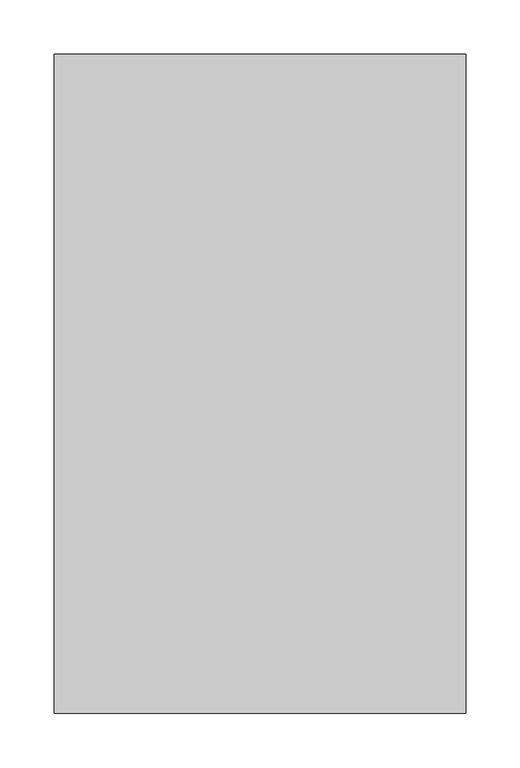
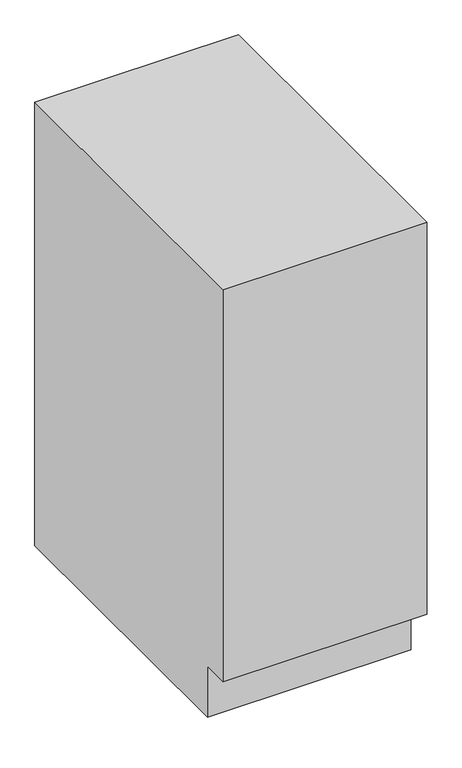
"""IFC4 building model written with IfcOpenShell, lengths in millimetres: furniture geometry, Cabinet, Base Integrated Trash Single-NON-COLLECTUS : -."""

import ifcopenshell
import ifcopenshell.guid

model = None  # the IFC model being written
_history = None  # IfcOwnerHistory: only IFC2X3 demands one
_inside = {}  # id of a spatial element -> (the spatial element, [elements in it])
_under = {}  # id of a project, library or spatial element -> (it, [spatial elements below it])
_declared = {}  # id of a project -> (the project, [libraries it declares])
_typed = {}  # id of a type object -> (the type object, [elements of that type])
_made_of = {}  # id of a material, layer set ... -> (it, [elements and type objects made of it])


def new_model(schema):
    """Start an empty IFC model of exactly this schema.

    Asked for "IFC4X3", IfcOpenShell would pick the latest addendum, in which some entities
    have other attributes; the version numbers below select the first issue.
    IFC2X3 requires an IfcOwnerHistory on every rooted entity: one is made here for all.
    """
    global model, _history
    if schema == "IFC4X3":
        model = ifcopenshell.file(schema_version=(4, 3, 0, 0))
    else:
        model = ifcopenshell.file(schema=schema)
    _inside.clear()
    _under.clear()
    _declared.clear()
    _typed.clear()
    _made_of.clear()
    _history = None
    if model.schema == "IFC2X3":
        org = make("IfcOrganization", Name="unknown")
        user = make(
            "IfcPersonAndOrganization",
            ThePerson=make("IfcPerson", FamilyName="unknown"),
            TheOrganization=org,
        )
        app = make(
            "IfcApplication",
            ApplicationDeveloper=org,
            Version="unknown",
            ApplicationFullName="unknown",
            ApplicationIdentifier="unknown",
        )
        _history = make(
            "IfcOwnerHistory",
            OwningUser=user,
            OwningApplication=app,
            ChangeAction="ADDED",
            CreationDate=0,
        )
    return model


def make(cls, **values):
    """One entity of the class cls with the attributes given. An attribute that is None is left unset."""
    return model.create_entity(
        cls, **{name: value for name, value in values.items() if value is not None}
    )


def rooted(cls, **values):
    """An entity with a GlobalId (a new one), such as an element, a storey or a relation."""
    return make(cls, GlobalId=ifcopenshell.guid.new(), OwnerHistory=_history, **values)


def si_unit(unit_type, name, prefix=None):
    """IfcSIUnit, for example si_unit("LENGTHUNIT", "METRE", prefix="MILLI")."""
    return make("IfcSIUnit", UnitType=unit_type, Prefix=prefix, Name=name)


def assignment(units):
    """IfcUnitAssignment: the units of a project."""
    return None if units is None else make("IfcUnitAssignment", Units=units)


def point(xyz):
    """IfcCartesianPoint."""
    return None if xyz is None else make("IfcCartesianPoint", Coordinates=xyz)


def direction(xyz):
    """IfcDirection."""
    return None if xyz is None else make("IfcDirection", DirectionRatios=xyz)


def frame(location, z_axis=None, x_axis=None):
    """IfcAxis2Placement3D, a coordinate frame: its origin and axes. An axis left out is left unset."""
    return make(
        "IfcAxis2Placement3D",
        Location=point(location),
        Axis=direction(z_axis),
        RefDirection=direction(x_axis),
    )


def origin():
    """The frame at (0, 0, 0) with its axes left unset."""
    return frame((0.0, 0.0, 0.0))


def place(relative_to, where):
    """IfcLocalPlacement: puts the frame where relative to a parent placement (None: the world)."""
    return make(
        "IfcLocalPlacement", PlacementRelTo=relative_to, RelativePlacement=where
    )


def context(
    kind, dimensions, precision=None, world=None, true_north=None, identifier=None
):
    """IfcGeometricRepresentationContext, for example the 3D "Model" context."""
    return make(
        "IfcGeometricRepresentationContext",
        ContextIdentifier=identifier,
        ContextType=kind,
        CoordinateSpaceDimension=dimensions,
        Precision=precision,
        WorldCoordinateSystem=world,
        TrueNorth=true_north,
    )


def project(units=None, contexts=None):
    """IfcProject with its units and contexts."""
    return rooted(
        "IfcProject",
        Name="project",
        RepresentationContexts=contexts,
        UnitsInContext=assignment(units),
    )


def spatial(cls, under=None, at=None, **own):
    """A site, building, storey or space (cls), placed at a placement, below another one or the project."""
    s = rooted(cls, ObjectPlacement=at, **own)
    if under is not None:
        _under.setdefault(under.id(), (under, []))[1].append(s)
    return s


def polyline(points):
    """IfcPolyline through the points."""
    return make("IfcPolyline", Points=[point(p) for p in points])


def outline(outer, holes=None, kind="AREA"):
    """IfcArbitraryClosedProfileDef: a profile drawn as a closed curve; with holes, ...WithVoids."""
    if holes is None:
        return make("IfcArbitraryClosedProfileDef", ProfileType=kind, OuterCurve=outer)
    return make(
        "IfcArbitraryProfileDefWithVoids",
        ProfileType=kind,
        OuterCurve=outer,
        InnerCurves=holes,
    )


def extrude(swept, where, along, depth):
    """IfcExtrudedAreaSolid: the profile swept, set in the frame where, extruded along a direction by depth."""
    return make(
        "IfcExtrudedAreaSolid",
        SweptArea=swept,
        Position=where,
        ExtrudedDirection=direction(along),
        Depth=depth,
    )


def shape(context_of_items, identifier, shape_type, items):
    """IfcShapeRepresentation: the items that make up one representation, for example the "Body"."""
    return make(
        "IfcShapeRepresentation",
        ContextOfItems=context_of_items,
        RepresentationIdentifier=identifier,
        RepresentationType=shape_type,
        Items=items,
    )


def source(mapping_origin, context_of_items, identifier, shape_type, items):
    """IfcRepresentationMap: a shape defined once, which mapped items show again and again."""
    return make(
        "IfcRepresentationMap",
        MappingOrigin=mapping_origin,
        MappedRepresentation=shape(context_of_items, identifier, shape_type, items),
    )


def transform(
    local_origin,
    x_axis=None,
    y_axis=None,
    z_axis=None,
    scale=None,
    scale2=None,
    scale3=None,
    uniform=True,
):
    """IfcCartesianTransformationOperator3D, or its non-uniform kind. x_axis, y_axis, z_axis: its Axis1, 2, 3."""
    if uniform:
        return make(
            "IfcCartesianTransformationOperator3D",
            Axis1=direction(x_axis),
            Axis2=direction(y_axis),
            LocalOrigin=point(local_origin),
            Scale=scale,
            Axis3=direction(z_axis),
        )
    return make(
        "IfcCartesianTransformationOperator3DnonUniform",
        Axis1=direction(x_axis),
        Axis2=direction(y_axis),
        LocalOrigin=point(local_origin),
        Scale=scale,
        Axis3=direction(z_axis),
        Scale2=scale2,
        Scale3=scale3,
    )


def mapped(mapping_source, mapping_target):
    """IfcMappedItem: shows the shape of a source again, moved by a transform."""
    return make(
        "IfcMappedItem", MappingSource=mapping_source, MappingTarget=mapping_target
    )


def made_of(thing, what):
    """Note that an element or type object is made of a material, layer set ...; save() writes the relation."""
    if what is not None:
        _made_of.setdefault(what.id(), (what, []))[1].append(thing)
    return thing


def element(
    cls,
    number,
    at=None,
    inside=None,
    cuts=None,
    type_object=None,
    material=None,
    context=None,
    identifier="Body",
    shape_type=None,
    held_by="IfcProductDefinitionShape",
    body=None,
    shapes=None,
    **own,
):
    """One element of the class cls, such as IfcWall. Its Tag is "e" and its number.

    at: its placement. inside: the storey or other place that contains it. cuts: it is an
    opening in that element (IfcRelVoidsElement). A single representation is given by context,
    identifier, shape_type and body (its items); several are given by shapes. held_by: the class
    of the entity that holds the representations. save() writes the other relations.
    """
    e = rooted(cls, Tag="e%d" % number, ObjectPlacement=at, **own)
    if body is not None:
        shapes = [shape(context, identifier, shape_type, body)]
    if shapes is not None:
        e.Representation = make(held_by, Representations=shapes)
    if inside is not None:
        _inside.setdefault(inside.id(), (inside, []))[1].append(e)
    if cuts is not None:
        rooted(
            "IfcRelVoidsElement", RelatingBuildingElement=cuts, RelatedOpeningElement=e
        )
    if type_object is not None:
        _typed.setdefault(type_object.id(), (type_object, []))[1].append(e)
    return made_of(e, material)


def aggregate(whole, parts):
    """IfcRelAggregates: a whole, such as a stair, and the parts it consists of."""
    return rooted("IfcRelAggregates", RelatingObject=whole, RelatedObjects=parts)


def save(model, path):
    """Write the relations noted so far, then the file.

    IfcRelAggregates (storeys below a building ...), IfcRelContainedInSpatialStructure (elements
    in a storey), IfcRelDefinesByType, IfcRelAssociatesMaterial and IfcRelDeclares: one each for
    every whole, place, type object, material and project.
    """
    for whole, parts in _under.values():
        aggregate(whole, parts)
    for where, things in _inside.values():
        rooted(
            "IfcRelContainedInSpatialStructure",
            RelatedElements=things,
            RelatingStructure=where,
        )
    for kind, things in _typed.values():
        rooted("IfcRelDefinesByType", RelatedObjects=things, RelatingType=kind)
    for what, things in _made_of.values():
        rooted("IfcRelAssociatesMaterial", RelatedObjects=things, RelatingMaterial=what)
    for by, libraries in _declared.values():
        rooted("IfcRelDeclares", RelatingContext=by, RelatedDefinitions=libraries)
    model.write(path)


def furniture_cb5fd4a6(model_context):
    return source(origin(), model_context, "Body", "SweptSolid", [
        extrude(outline(polyline([(1384.3, 876.2982474), (1993.8987808, 876.2982474), (1993.8987808, 0.0), (1435.1, 0.0), (1435.1, 101.6), (1384.3, 101.6), (1384.3, 876.2982474)])), frame((114.3, 0.0, 0.0), z_axis=(1.0, 0.0, 0.0), x_axis=(0.0, 1.0, 0.0)), (0.0, 0.0, 1.0), 380.999238),
    ])


if __name__ == "__main__":
    model = new_model("IFC4")
    model_context = context("Model", 3, world=origin())
    ifc_project = project(units=[si_unit("LENGTHUNIT", "METRE", prefix="MILLI")], contexts=[model_context])
    site = spatial("IfcSite", under=ifc_project)
    building = spatial("IfcBuilding", under=site)
    placement = place(None, origin())
    furniture_shape = furniture_cb5fd4a6(model_context)
    element("IfcFurniture", 1, ObjectType="Cabinet, Base Integrated Trash Single-NON-COLLECTUS : -", at=placement, inside=building, context=model_context, shape_type="MappedRepresentation", body=[
        mapped(furniture_shape, transform((0.0, 0.0, 0.0), x_axis=(1.0, 0.0, 0.0), y_axis=(0.0, 1.0, 0.0), z_axis=(0.0, 0.0, 1.0))),
    ])
    save(model, "model.ifc")

# Revit data of these elements
# Type "Cabinet, Base Integrated Trash Single-NON-COLLECTUS : -"
#   External ID [instance default] = ""
#   Width Reporting [instance default] = 381 mm
#   Width [instance default] = 381 mm
#   Toe Kick Height = 101.6 mm
#   Toe Kick Depth = 50.8 mm
#   Height of Drawer = 152.4 mm
#   Height Reporting [instance default] = 825.5 mm
#   Height [instance default] = 825.5 mm
#   Depth Reporting [instance default] = 609.6 mm
#   Depth [instance default] = 609.6 mm
#   Material = White
#   Default Elevation = 0
# Element 1 (IfcFurniture, "Cabinet, Base Integrated Trash Single-NON-COLLECTUS : -")
#   Width Reporting = 380.999 mm
#   Width = 380.999 mm
#   Height Reporting = 876.298 mm
#   Height = 876.298 mm
#   Depth Reporting = 609.599 mm
#   Depth = 609.599 mm
#   Materials on its faces: "White"
# Materials
#   "White": class "Generic", colour RGB 255 255 255, transparency 0, Cost = 0
